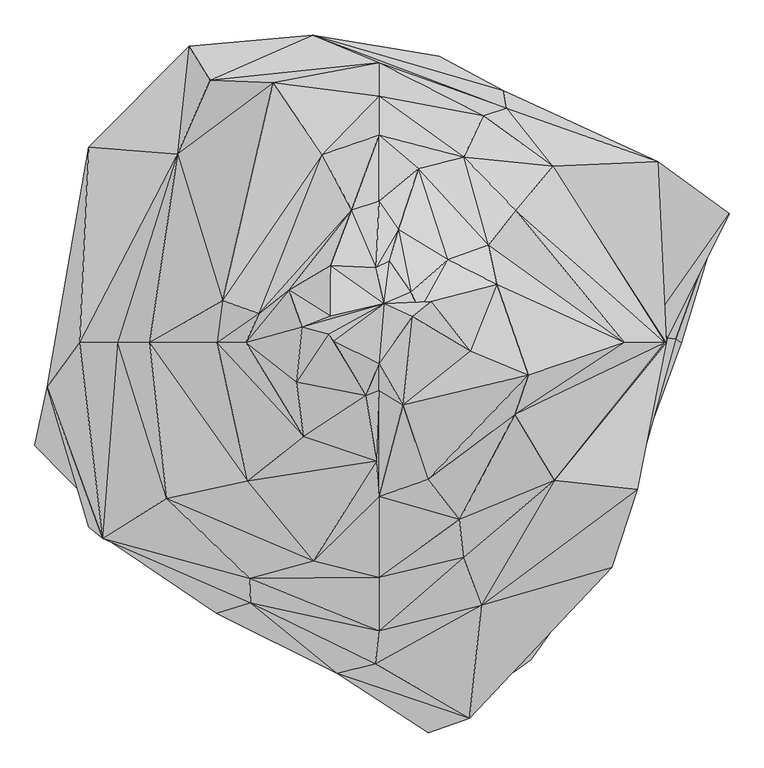
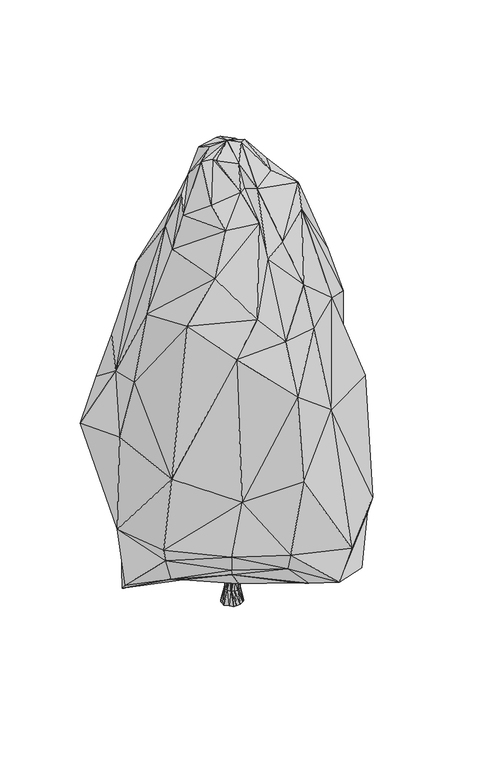
"""IFC4 building model written with IfcOpenShell, lengths in millimetres: geographic element geometry, Enscape AssetDefinition - Coniferous Tree 006 Pine : Enscape AssetDefinition - Coniferous Tree 006 Pine."""

from ifc_helpers import new_model, si_unit, origin, place, context, project, spatial, faceted_brep, source, transform, mapped, element, save


def geographic_element_220c0fd0(model_context):
    return source(origin(), model_context, "Body", "Brep", [
        faceted_brep([(382.163763, 91.6514024, -68.5002655), (-22.9553711, -3.1674753, -68.7730536), (237.0086759, 234.688431, -71.9918683), (378.2389462, -3.1674753, -68.7730536), (48.4780967, 358.6789072, -82.5051889), (-288.6125445, 304.8959672, -68.7730536), (-428.7452102, 105.8360413, -68.7730536), (-433.7836802, -3.1674753, -68.7730536), (-438.9889836, -99.8284221, -84.2734575), (-290.4289365, -242.1594411, -92.1038911), (-187.827751, -374.9398589, -84.0584412), (-55.801481, -344.6579278, -93.4838504), (94.94403, -367.9919541, -71.40138), (331.8596482, -208.5944563, -69.3410784), (-285.708189, -112.1677756, 506.2280297), (-206.2196583, -208.026439, 506.2280297), (-182.3079437, -242.072776, 506.2280297), (-78.2979354, -279.9316645, 506.2280297), (-197.2403228, -208.026439, 1081.2259912), (-182.3079437, -229.300186, 1081.2259912), (-78.2979354, -267.1590745, 1081.2259912), (-261.4499032, -133.3548725, 1081.2259912), (-170.7131267, -208.026439, 1656.2269926), (-135.6205642, -235.9528393, 1656.2269926), (32.3871933, -279.9316645, 506.2280297), (32.3871933, -267.1590745, 1081.2259912), (-78.2979354, -273.811698, 1656.2269926), (242.2460765, -283.7217152, -73.3236894), (102.8482765, -242.072776, 506.2280297), (98.8143161, -229.300186, 1081.2259912), (32.3871933, -273.811698, 1656.2269926), (-149.7763395, -237.9393429, 2231.2281132), (-78.2979354, -275.7982016, 2231.2281132), (98.3201042, -235.9528393, 1656.2269926), (32.3871933, -275.7982016, 2231.2281132), (66.5972158, -237.9393429, 2231.2281132), (-138.0724013, -239.9867922, 2806.2257767), (-78.2979354, -277.8456807, 2806.2257767), (32.3871933, -277.8456807, 2806.2257767), (151.3841301, -208.026439, 2231.2281132), (63.766703, -239.9867922, 2806.2257767), (183.1070334, -208.026439, 1656.2269926), (238.4496033, -112.1709943, 1656.2269926), (206.726715, -112.1709943, 2231.2281132), (148.5536397, -208.026439, 2806.2257767), (183.6012453, -208.026439, 1081.2259912), (238.9438152, -112.1709943, 1081.2259912), (234.2327237, -3.1674753, 1656.2269926), (225.9594053, -3.1674753, 2231.2281132), (174.8947054, -112.1709943, 2806.2257767), (200.812161, -3.1674753, 2806.2257767), (148.707673, 85.5988562, 2806.2257767), (-22.9553711, -3.1674753, 2806.2257767), (165.8062786, 105.8360413, 2231.2281132), (118.9680621, 140.2161419, 2231.2281132), (108.0054566, 117.7389398, 2806.2257767), (176.781714, 105.8360413, 1656.2269926), (115.6946868, 166.8685079, 1656.2269926), (98.1692746, 168.3190763, 1656.2269926), (95.4671353, 145.7584351, 2231.2281132), (73.0156004, 148.0273157, 2806.2257767), (32.3871933, 183.6140901, 2231.2281132), (136.3971978, 184.702009, 1081.2259912), (32.3871933, 222.5576639, 1081.2259912), (32.3871933, 206.1747313, 1656.2269926), (-78.2979354, 206.1747313, 1656.2269926), (-78.2979354, 183.6140901, 2231.2281132), (32.3871933, 165.2286053, 2806.2257767), (-54.0749319, 169.8498577, 2806.2257767), (-131.2881708, 197.5997537, 1656.2269926), (-119.7607368, 168.6271429, 2231.2281132), (-102.2385359, 157.2698057, 2806.2257767), (-188.8418645, 166.8685079, 1656.2269926), (-162.7832055, 140.2161419, 2231.2281132), (-120.190762, 221.3702649, 1081.2259912), (-178.3574373, 203.1163573, 1081.2259912), (-235.9977663, 114.3917516, 1081.2259912), (-244.1844344, 105.8360413, 1656.2269926), (-218.1257606, 105.8360413, 2231.2281132), (-138.7431175, 133.8715702, 2806.2257767), (-179.7662675, 105.8360413, 2806.2257767), (-263.4043097, -3.1674753, 1656.2269926), (-237.3456359, -3.1674753, 2231.2281132), (-297.5758016, -25.6543029, 1081.2259912), (-257.0853829, -136.9491816, 1656.2269926), (-265.0666535, -112.1677756, 2231.2281132), (-198.986128, -3.1674753, 2806.2257767), (-242.2011495, -112.1677756, 2806.2257767), (-142.6198334, -208.026439, 2806.2257767), (-177.1924943, -208.026439, 2231.2281132), (-304.9280941, -3.1674753, 506.2280297), (-264.8612559, 105.8360413, 506.2280297), (-209.5187008, 201.6914785, 506.2280297), (-142.555654, 232.5382531, 506.2280297), (-373.4026551, 201.6914785, -68.7730536), (-78.2979354, 252.7433634, 506.2280297), (-78.2979354, 222.5576639, 1081.2259912), (32.3871933, 252.7433634, 506.2280297), (-184.6025288, 342.7516222, -68.7730536), (136.3971978, 214.8876935, 506.2280297), (137.2027099, 321.9624758, -69.5785508), (177.7637154, 163.3480191, 506.2280297), (173.2259244, 149.3527293, 1081.2259912), (241.5689379, 77.9128298, 506.2280297), (219.184801, 105.8360413, 1081.2259912), (244.636938, -3.1674753, 506.2280297), (238.4078801, -3.1674753, 1081.2259912), (242.9777682, -112.1709943, 506.2280297), (187.6351982, -208.026439, 506.2280297), (359.0158522, -112.1709943, -68.7730536)], [[[0, 1, 2]], [[3, 1, 0]], [[1, 4, 2]], [[5, 4, 1]], [[6, 5, 1]], [[1, 7, 6]], [[8, 7, 1]], [[1, 9, 8]], [[10, 9, 1]], [[1, 11, 10]], [[12, 11, 1]], [[13, 12, 1]], [[1, 3, 13]], [[14, 9, 15]], [[8, 9, 14]], [[10, 15, 9]], [[16, 15, 10]], [[10, 11, 16]], [[16, 11, 17]], [[11, 12, 17]], [[18, 16, 19]], [[15, 16, 18]], [[20, 16, 17]], [[19, 16, 20]], [[18, 14, 15]], [[21, 14, 18]], [[22, 21, 18]], [[19, 22, 18]], [[23, 22, 19]], [[19, 20, 23]], [[20, 24, 25]], [[17, 24, 20]], [[23, 20, 26]], [[20, 25, 26]], [[17, 12, 24]], [[24, 27, 28]], [[12, 27, 24]], [[24, 28, 25]], [[25, 28, 29]], [[26, 25, 30]], [[29, 30, 25]], [[26, 31, 23]], [[32, 31, 26]], [[26, 30, 32]], [[33, 30, 29]], [[32, 30, 34]], [[35, 30, 33]], [[34, 30, 35]], [[36, 32, 37]], [[31, 32, 36]], [[34, 37, 32]], [[38, 37, 34]], [[34, 35, 38]], [[33, 39, 35]], [[38, 35, 40]], [[39, 40, 35]], [[33, 29, 41]], [[41, 39, 33]], [[42, 39, 41]], [[43, 39, 42]], [[44, 40, 39]], [[43, 44, 39]], [[41, 29, 45]], [[41, 46, 42]], [[45, 46, 41]], [[42, 46, 47]], [[42, 47, 43]], [[43, 47, 48]], [[49, 44, 43]], [[48, 49, 43]], [[49, 40, 44]], [[50, 49, 48]], [[49, 51, 52]], [[50, 51, 49]], [[52, 40, 49]], [[48, 47, 53]], [[53, 50, 48]], [[51, 50, 53]], [[54, 51, 53]], [[55, 51, 54]], [[51, 55, 52]], [[53, 47, 56]], [[53, 57, 54]], [[56, 57, 53]], [[58, 54, 57]], [[59, 54, 58]], [[54, 59, 55]], [[55, 59, 60]], [[52, 55, 60]], [[58, 61, 59]], [[61, 60, 59]], [[57, 62, 58]], [[58, 63, 64]], [[62, 63, 58]], [[64, 61, 58]], [[61, 65, 66]], [[64, 65, 61]], [[67, 60, 61]], [[61, 66, 67]], [[68, 60, 67]], [[52, 60, 68]], [[67, 66, 68]], [[69, 66, 65]], [[70, 66, 69]], [[70, 68, 66]], [[71, 68, 70]], [[71, 52, 68]], [[72, 70, 69]], [[73, 70, 72]], [[70, 73, 71]], [[65, 74, 69]], [[69, 74, 72]], [[72, 74, 75]], [[72, 76, 77]], [[75, 76, 72]], [[77, 73, 72]], [[78, 73, 77]], [[71, 73, 79]], [[73, 78, 79]], [[79, 52, 71]], [[79, 78, 80]], [[79, 80, 52]], [[81, 78, 77]], [[82, 78, 81]], [[78, 82, 80]], [[77, 83, 81]], [[76, 83, 77]], [[81, 83, 84]], [[85, 81, 84]], [[82, 81, 85]], [[80, 82, 86]], [[82, 85, 86]], [[52, 80, 86]], [[86, 85, 87]], [[88, 86, 87]], [[52, 86, 88]], [[85, 22, 89]], [[84, 22, 85]], [[89, 87, 85]], [[84, 83, 21]], [[84, 21, 22]], [[22, 23, 89]], [[89, 23, 31]], [[88, 87, 89]], [[31, 88, 89]], [[36, 88, 31]], [[37, 88, 36]], [[52, 88, 37]], [[40, 37, 38]], [[52, 37, 40]], [[83, 14, 21]], [[90, 8, 14]], [[90, 14, 83]], [[76, 90, 83]], [[91, 7, 90]], [[7, 8, 90]], [[91, 90, 76]], [[76, 75, 91]], [[92, 6, 91]], [[6, 7, 91]], [[91, 75, 92]], [[74, 92, 75]], [[93, 94, 92]], [[94, 6, 92]], [[93, 92, 74]], [[94, 5, 6]], [[5, 94, 93]], [[95, 5, 93]], [[93, 74, 95]], [[95, 74, 96]], [[96, 74, 65]], [[95, 97, 98]], [[98, 5, 95]], [[63, 95, 96]], [[97, 95, 63]], [[98, 4, 5]], [[98, 97, 4]], [[99, 4, 97]], [[62, 97, 63]], [[99, 97, 62]], [[96, 64, 63]], [[65, 64, 96]], [[99, 2, 100]], [[101, 2, 99]], [[100, 4, 99]], [[102, 99, 62]], [[101, 99, 102]], [[2, 4, 100]], [[101, 0, 2]], [[103, 0, 101]], [[102, 103, 101]], [[104, 103, 102]], [[57, 104, 102]], [[102, 62, 57]], [[105, 0, 103]], [[106, 103, 104]], [[105, 103, 106]], [[3, 0, 105]], [[107, 3, 105]], [[46, 105, 106]], [[107, 105, 46]], [[106, 104, 47]], [[47, 46, 106]], [[47, 104, 56]], [[56, 104, 57]], [[46, 45, 107]], [[29, 108, 45]], [[107, 45, 108]], [[28, 13, 108]], [[13, 107, 108]], [[28, 108, 29]], [[27, 12, 13]], [[13, 3, 109]], [[27, 13, 28]], [[109, 107, 13]], [[109, 3, 107]]]),
        faceted_brep([(426.6528189, 564.5583272, 19617.1035767), (-2.5416825, 381.4128339, 19780.7064056), (555.0431013, 261.2797916, 19595.8957672), (87.992914, 1050.2314568, 19526.7543793), (-125.0719577, 951.7253041, 19619.304657), (-846.5182185, 981.6253185, 19435.3561401), (-842.8276181, 185.7642382, 19906.5189362), (-1297.0795631, 13.026122, 19517.4732208), (-876.9093156, -94.4337696, 19547.0523834), (-797.4689007, -208.7228298, 19514.7762299), (-83.9525387, -560.8421564, 19356.6951752), (449.1268098, 178.3798933, 19650.7320404), (736.2278104, 411.4990234, 19547.6570129), (-282.078594, -1069.5186853, 18486.240387), (-1383.0891848, -857.0604324, 18172.4834442), (-83.9525387, -988.0020022, 18546.0605621), (-1271.181345, -1710.0163698, 17535.0589752), (-123.2876405, -2098.9353657, 17707.3745728), (-2180.2630424, -233.6839437, 17632.4748993), (-2635.8401775, -233.6839437, 16304.8439026), (-2151.2293816, -2414.1585827, 16174.829483), (-83.9525387, -2660.8588696, 16461.8167877), (-1113.1060123, -3673.8414764, 14779.8252106), (-3699.007988, -233.6839437, 13853.4040451), (-3430.6614399, -2689.5682812, 14717.9365158), (-1975.692749, 226.2514532, 18230.4344177), (-2548.9385128, 432.1887195, 16915.4987335), (-3260.4489326, 2745.4018593, 9411.5829468), (-4203.4258842, -233.6839437, 11052.3967743), (-2125.8027554, -3951.5297413, 13569.483757), (-4441.3332939, -3317.861557, 8759.3698502), (-4805.9425354, -233.6839437, 8850.9759903), (-2107.7799797, -4341.1903381, 7558.7835312), (-5319.9243546, -934.4277382, 5446.8507767), (-4665.8034325, -3135.8168125, 5639.9388313), (-83.9525387, -3935.4259968, 13618.4015274), (-83.9525387, -4779.0527344, 11699.8653412), (1248.7618923, -3618.2837486, 13557.7859879), (-136.8400753, -5300.5819321, 8346.6768265), (1532.6441526, -4375.9713173, 10346.6272354), (1190.8166409, -3024.8908997, 15116.5370941), (2687.7038479, -2409.9481106, 13650.7568359), (3995.9001541, -2544.8596478, 9891.6826248), (1350.7020473, -6157.389164, 5446.8507767), (3593.5988426, -3780.6210518, 5446.8507767), (-745.0306416, -5450.0889778, 5446.8507767), (703.2501698, -6384.9658966, 4321.6657639), (-2642.4446106, -4504.6887398, 5446.8507767), (-745.0306416, -5239.9058342, 4731.2679291), (-4464.4842148, -2921.4971066, 4962.9750252), (-2548.5081673, -4322.6671219, 4731.2679291), (-2249.0999699, -3864.6793365, 4154.5562744), (-83.9525387, -5575.6392479, 4064.4483566), (-4219.1700935, -2904.661417, 4064.4483566), (-5511.7921829, -1853.7561893, 3627.4621487), (-5238.6322021, -1153.0122757, 2960.6425762), (-3460.3464603, -2414.5276546, 3491.8382168), (-3490.9300804, 2056.4618111, 4731.2679291), (-4660.9258652, 2850.4936695, 7541.4409637), (-3762.0074749, 2722.7835655, 5446.8507767), (-2909.3663692, 3684.2262745, 5446.8507767), (-2138.9443874, 2996.8168736, 4731.2679291), (-2950.3154755, 1747.3585606, 4064.4483566), (-3078.7539482, 4446.7859268, 8073.9364624), (-1128.4556389, 4623.7277985, 7984.9839211), (866.3734794, 4285.9277725, 5446.8507767), (-2746.8268871, 3909.3577862, 10135.635376), (-1752.2941828, 3867.3493862, 12950.0360489), (-83.9525387, 4187.5886917, 9583.4712982), (1931.447506, 3472.1112251, 12317.0022964), (1886.1657381, 3746.2472916, 5616.3158417), (879.2455792, 3946.9151497, 4731.2679291), (1874.9047518, 3499.7522831, 4753.5877228), (1981.2414646, 3296.4208126, 4373.3911514), (-8.122473, 3264.6818161, 4064.4483566), (-1671.3488102, 2603.918314, 4064.4483566), (-111.1023277, 2467.6012993, 3491.8382168), (4051.2685776, 2437.2935295, 4064.4483566), (1814.1611814, 3249.2585182, 3491.8382168), (5281.9142342, 1700.8990049, 4731.2679291), (4690.9894943, -233.6839437, 4064.4483566), (3292.4413681, 1947.1597672, 3491.8382168), (1294.4544554, 2437.2935295, 3052.4578094), (-73.849991, 2154.97756, 3052.4578094), (-1156.7060947, 1737.5576496, 3491.8382168), (-1321.2159872, 1925.8826971, 3052.4578094), (-83.9525387, 1362.8038168, 2776.2551308), (2303.5185337, 1308.4048033, 3052.4578094), (629.5638084, 1148.9143372, 2776.2551308), (3814.7733212, -233.6839437, 3491.8382168), (2672.8613377, -233.6839437, 3052.4578094), (1151.8956423, 564.5583272, 2776.2551308), (-83.9525387, -233.6839437, 2682.046175), (-797.465682, 1148.9143372, 2776.2551308), (-1554.00455, 1273.6042738, 3052.4578094), (-1319.7973967, 564.5583272, 2776.2551308), (-2840.7633305, -233.6839437, 3052.4578094), (-1510.9820366, -233.6839437, 2776.2551308), (-2385.7989311, 1493.6652184, 3491.8382168), (-4767.9009438, -834.4324231, 2706.612587), (-2471.4233875, -1775.7726908, 3052.4578094), (-1319.7973967, -1031.929493, 2776.2551308), (-797.4689007, -1616.2822247, 2776.2551308), (-1462.3594284, -2904.661417, 3052.4578094), (-1930.333972, -3783.4579945, 3594.8181152), (-83.9525387, -3317.861557, 3052.4578094), (-83.9525387, -1830.1717043, 2776.2551308), (1294.4544554, -2904.661417, 3052.4578094), (629.5638084, -1616.2853241, 2776.2551308), (-83.9525387, -4595.3712463, 3491.8382168), (1865.408659, -4011.0187531, 3491.8382168), (2316.3905144, -5233.1476212, 3691.2546158), (3376.9683838, -3618.6304092, 4064.4483566), (3292.4413681, -2414.5307541, 3491.8382168), (2303.5185337, -1775.7759094, 3052.4578094), (3430.8958054, -3675.5328178, 4731.2679291), (4605.3133011, -171.0179895, 4731.2679291), (4471.1112976, -158.0560505, 5446.8507767), (4307.8689575, 190.494597, 6404.3655396), (5444.6172714, 1805.9905767, 5446.8507767), (4322.9045868, 2621.5946674, 11092.9937363), (4454.4491768, -233.6839437, 8866.6524887), (2661.8540287, 2549.2017269, 14702.712059), (4428.5383224, -233.6839437, 12026.766777), (2081.4323425, 1847.7196693, 17182.9471588), (1257.1153641, 2694.9021816, 17175.8804321), (1565.2239323, 3353.3358574, 14745.2173233), (3789.9243832, -233.6839437, 14108.1342697), (2063.4000301, -1363.9335632, 17101.9077301), (688.8568997, -2393.914938, 16781.7668915), (2277.992487, -742.9992557, 17827.2571564), (1644.4268227, 1308.2411289, 17544.3077087), (1780.0345421, 680.506587, 18216.4974213), (1006.1628819, 1078.1419277, 18460.6304169), (538.8334394, 2512.3279095, 17458.3091736), (1364.7197485, -363.6852205, 18439.1479492), (295.7722545, -1219.882369, 18540.0447845), (228.0806899, 1553.5135269, 18752.7065277), (-83.9525387, 2000.2913475, 18096.5957642), (-514.613688, 1859.5167398, 18085.8325958), (-83.9525387, 3041.2480831, 16153.1772614), (-1497.1183538, 597.43011, 18716.2075043), (-976.564467, 2735.6684208, 15758.2159042), (-83.9525387, 3654.2782784, 14337.8000259), (1151.8956423, -1031.929493, 2776.2551308), (1343.080163, -233.6839437, 2776.2551308)], [[[0, 1, 2]], [[3, 1, 0]], [[4, 1, 3]], [[5, 1, 4]], [[6, 1, 5]], [[7, 1, 6]], [[8, 1, 7]], [[9, 1, 8]], [[10, 1, 9]], [[11, 1, 10]], [[12, 1, 11]], [[2, 1, 12]], [[9, 8, 13]], [[9, 13, 10]], [[8, 7, 14]], [[13, 8, 14]], [[10, 13, 15]], [[13, 16, 17]], [[14, 16, 13]], [[13, 17, 15]], [[14, 7, 18]], [[14, 18, 16]], [[16, 18, 19]], [[16, 19, 20]], [[16, 20, 17]], [[15, 17, 21]], [[17, 20, 22]], [[17, 22, 21]], [[20, 19, 23]], [[20, 23, 24]], [[20, 24, 22]], [[18, 25, 19]], [[19, 26, 23]], [[25, 26, 19]], [[23, 27, 28]], [[26, 27, 23]], [[24, 23, 28]], [[22, 24, 29]], [[24, 28, 30]], [[24, 30, 29]], [[28, 27, 31]], [[30, 28, 31]], [[29, 30, 32]], [[30, 33, 34]], [[31, 33, 30]], [[30, 34, 32]], [[35, 29, 36]], [[22, 29, 35]], [[29, 32, 36]], [[37, 35, 36]], [[36, 32, 38]], [[39, 36, 38]], [[37, 36, 39]], [[21, 22, 35]], [[40, 21, 35]], [[40, 35, 37]], [[41, 40, 37]], [[37, 39, 41]], [[41, 39, 42]], [[39, 38, 43]], [[39, 44, 42]], [[43, 44, 39]], [[38, 32, 45]], [[43, 38, 45]], [[45, 46, 43]], [[43, 46, 44]], [[45, 32, 47]], [[45, 47, 48]], [[48, 46, 45]], [[32, 34, 47]], [[47, 49, 50]], [[34, 49, 47]], [[48, 47, 50]], [[48, 51, 52]], [[50, 51, 48]], [[48, 52, 46]], [[50, 53, 51]], [[49, 53, 50]], [[49, 33, 54]], [[34, 33, 49]], [[49, 54, 53]], [[53, 54, 55]], [[53, 55, 56]], [[53, 56, 51]], [[33, 57, 54]], [[57, 55, 54]], [[33, 58, 59]], [[31, 58, 33]], [[59, 57, 33]], [[60, 57, 59]], [[61, 57, 60]], [[61, 62, 57]], [[62, 55, 57]], [[58, 60, 59]], [[27, 63, 58]], [[31, 27, 58]], [[63, 60, 58]], [[60, 64, 65]], [[63, 64, 60]], [[65, 61, 60]], [[66, 64, 63]], [[66, 63, 27]], [[27, 67, 66]], [[26, 67, 27]], [[67, 68, 66]], [[68, 64, 66]], [[64, 68, 69]], [[64, 70, 65]], [[69, 70, 64]], [[65, 70, 71]], [[71, 61, 65]], [[71, 70, 72]], [[71, 73, 74]], [[72, 73, 71]], [[71, 74, 61]], [[61, 74, 75]], [[75, 62, 61]], [[74, 73, 76]], [[74, 76, 75]], [[72, 77, 73]], [[73, 77, 78]], [[76, 73, 78]], [[70, 79, 72]], [[79, 77, 72]], [[79, 80, 77]], [[77, 80, 81]], [[78, 77, 81]], [[78, 81, 82]], [[83, 78, 82]], [[76, 78, 83]], [[75, 76, 84]], [[76, 83, 84]], [[84, 83, 85]], [[83, 82, 86]], [[83, 86, 85]], [[82, 81, 87]], [[82, 87, 88]], [[86, 82, 88]], [[81, 80, 89]], [[81, 89, 87]], [[87, 89, 90]], [[87, 90, 91]], [[88, 87, 91]], [[88, 91, 92]], [[86, 88, 92]], [[85, 86, 93]], [[93, 86, 92]], [[94, 93, 95]], [[85, 93, 94]], [[95, 93, 92]], [[96, 95, 97]], [[94, 95, 96]], [[97, 95, 92]], [[98, 85, 94]], [[99, 94, 96]], [[98, 94, 99]], [[100, 99, 96]], [[101, 96, 97]], [[100, 96, 101]], [[101, 97, 92]], [[102, 100, 101]], [[102, 101, 92]], [[56, 99, 100]], [[103, 56, 100]], [[103, 100, 102]], [[55, 98, 99]], [[56, 55, 99]], [[51, 56, 104]], [[104, 56, 103]], [[105, 104, 103]], [[106, 103, 102]], [[105, 103, 106]], [[106, 102, 92]], [[107, 106, 108]], [[105, 106, 107]], [[108, 106, 92]], [[109, 104, 105]], [[110, 105, 107]], [[109, 105, 110]], [[109, 51, 104]], [[52, 51, 109]], [[111, 109, 110]], [[52, 109, 111]], [[112, 110, 113]], [[111, 110, 112]], [[110, 107, 113]], [[113, 107, 114]], [[107, 108, 114]], [[80, 113, 89]], [[112, 113, 80]], [[113, 114, 89]], [[115, 111, 112]], [[112, 80, 115]], [[46, 52, 111]], [[46, 111, 115]], [[44, 46, 115]], [[115, 116, 44]], [[115, 80, 116]], [[116, 80, 79]], [[79, 117, 116]], [[44, 116, 117]], [[118, 44, 117]], [[42, 44, 118]], [[119, 118, 117]], [[119, 117, 79]], [[119, 79, 70]], [[120, 118, 119]], [[70, 120, 119]], [[120, 121, 118]], [[121, 42, 118]], [[41, 42, 121]], [[122, 123, 121]], [[123, 41, 121]], [[122, 121, 120]], [[69, 122, 120]], [[69, 120, 70]], [[124, 123, 122]], [[125, 122, 126]], [[124, 122, 125]], [[126, 122, 69]], [[124, 127, 123]], [[127, 128, 123]], [[128, 41, 123]], [[128, 40, 41]], [[128, 129, 40]], [[130, 129, 128]], [[130, 128, 127]], [[131, 132, 127]], [[132, 130, 127]], [[131, 127, 124]], [[124, 125, 131]], [[133, 132, 131]], [[134, 133, 131]], [[131, 125, 134]], [[133, 2, 132]], [[132, 12, 135]], [[2, 12, 132]], [[135, 130, 132]], [[130, 136, 129]], [[135, 136, 130]], [[135, 11, 136]], [[12, 11, 135]], [[136, 10, 15]], [[11, 10, 136]], [[136, 21, 129]], [[15, 21, 136]], [[129, 21, 40]], [[0, 2, 133]], [[0, 137, 3]], [[133, 137, 0]], [[4, 137, 138]], [[3, 137, 4]], [[137, 133, 134]], [[137, 134, 138]], [[138, 139, 4]], [[138, 134, 140]], [[138, 140, 139]], [[4, 139, 5]], [[139, 141, 5]], [[139, 140, 142]], [[25, 139, 142]], [[141, 139, 25]], [[140, 125, 143]], [[134, 125, 140]], [[140, 143, 142]], [[142, 143, 67]], [[26, 142, 67]], [[25, 142, 26]], [[141, 25, 18]], [[7, 141, 18]], [[6, 141, 7]], [[5, 141, 6]], [[143, 68, 67]], [[143, 126, 68]], [[125, 126, 143]], [[69, 68, 126]], [[89, 114, 90]], [[114, 108, 144]], [[114, 144, 90]], [[91, 90, 145]], [[90, 144, 145]], [[144, 108, 92]], [[145, 144, 92]], [[91, 145, 92]], [[62, 98, 55]], [[62, 84, 98]], [[84, 85, 98]], [[75, 84, 62]]]),
    ])


if __name__ == "__main__":
    model = new_model("IFC4")
    model_context = context("Model", 3, world=origin())
    ifc_project = project(units=[si_unit("LENGTHUNIT", "METRE", prefix="MILLI")], contexts=[model_context])
    site = spatial("IfcSite", under=ifc_project)
    building = spatial("IfcBuilding", under=site)
    placement = place(None, origin())
    geographic_element_shape = geographic_element_220c0fd0(model_context)
    element("IfcGeographicElement", 1, ObjectType="Enscape AssetDefinition - Coniferous Tree 006 Pine : Enscape AssetDefinition - Coniferous Tree 006 Pine", at=placement, inside=building, context=model_context, shape_type="MappedRepresentation", body=[
        mapped(geographic_element_shape, transform((0.0, 0.0, 0.0), x_axis=(1.0, 0.0, 0.0), y_axis=(0.0, 1.0, 0.0), z_axis=(0.0, 0.0, 1.0))),
    ])
    save(model, "model.ifc")

# Revit data of these elements
# Type "Enscape AssetDefinition - Coniferous Tree 006 Pine : Enscape AssetDefinition - Coniferous Tree 006 Pine"
#   EnscapeAssetSource = "REMOTE"
#   EnscapeAssetId = "43d19a9d-9f11-4a69-a6eb-d063c6ff2aee"
#   Height = 19906.519 mm
#   EnscapeNativeAssetHeight = 19906.519 mm
#   Default Elevation = 0
